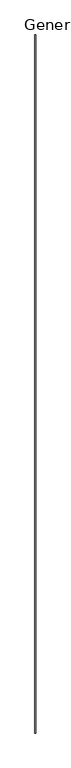
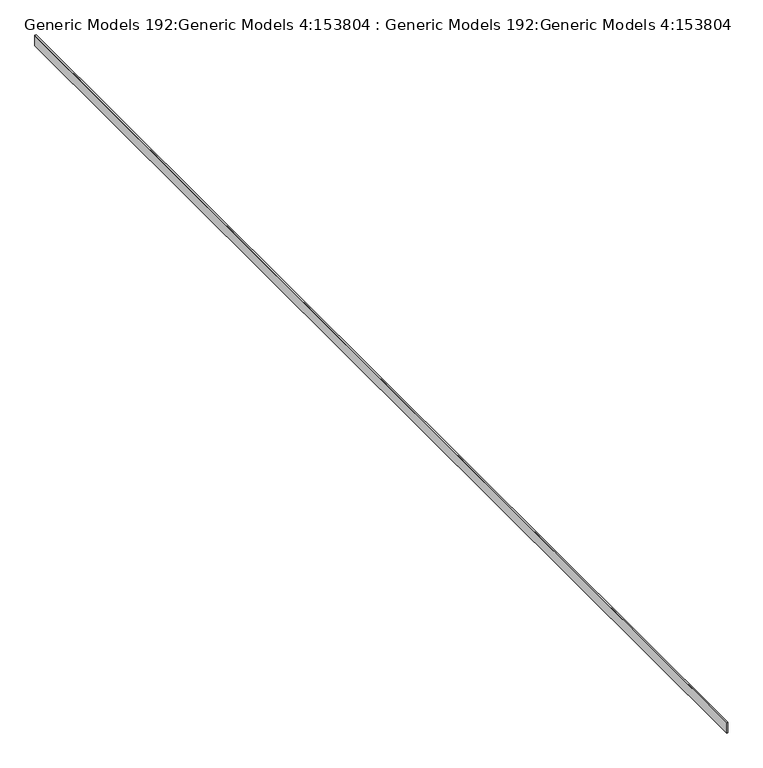
"""IFC4 building model written with IfcOpenShell, lengths in millimetres: proxy geometry, Generic Models 192:Generic Models 4:153804 : Generic Models 192:Generic Models 4:153804."""

import ifcopenshell
import ifcopenshell.guid

model = None  # the IFC model being written
_history = None  # IfcOwnerHistory: only IFC2X3 demands one
_inside = {}  # id of a spatial element -> (the spatial element, [elements in it])
_under = {}  # id of a project, library or spatial element -> (it, [spatial elements below it])
_declared = {}  # id of a project -> (the project, [libraries it declares])
_typed = {}  # id of a type object -> (the type object, [elements of that type])
_made_of = {}  # id of a material, layer set ... -> (it, [elements and type objects made of it])


def new_model(schema):
    """Start an empty IFC model of exactly this schema.

    Asked for "IFC4X3", IfcOpenShell would pick the latest addendum, in which some entities
    have other attributes; the version numbers below select the first issue.
    IFC2X3 requires an IfcOwnerHistory on every rooted entity: one is made here for all.
    """
    global model, _history
    if schema == "IFC4X3":
        model = ifcopenshell.file(schema_version=(4, 3, 0, 0))
    else:
        model = ifcopenshell.file(schema=schema)
    _inside.clear()
    _under.clear()
    _declared.clear()
    _typed.clear()
    _made_of.clear()
    _history = None
    if model.schema == "IFC2X3":
        org = make("IfcOrganization", Name="unknown")
        user = make(
            "IfcPersonAndOrganization",
            ThePerson=make("IfcPerson", FamilyName="unknown"),
            TheOrganization=org,
        )
        app = make(
            "IfcApplication",
            ApplicationDeveloper=org,
            Version="unknown",
            ApplicationFullName="unknown",
            ApplicationIdentifier="unknown",
        )
        _history = make(
            "IfcOwnerHistory",
            OwningUser=user,
            OwningApplication=app,
            ChangeAction="ADDED",
            CreationDate=0,
        )
    return model


def make(cls, **values):
    """One entity of the class cls with the attributes given. An attribute that is None is left unset."""
    return model.create_entity(
        cls, **{name: value for name, value in values.items() if value is not None}
    )


def rooted(cls, **values):
    """An entity with a GlobalId (a new one), such as an element, a storey or a relation."""
    return make(cls, GlobalId=ifcopenshell.guid.new(), OwnerHistory=_history, **values)


def si_unit(unit_type, name, prefix=None):
    """IfcSIUnit, for example si_unit("LENGTHUNIT", "METRE", prefix="MILLI")."""
    return make("IfcSIUnit", UnitType=unit_type, Prefix=prefix, Name=name)


def assignment(units):
    """IfcUnitAssignment: the units of a project."""
    return None if units is None else make("IfcUnitAssignment", Units=units)


def point(xyz):
    """IfcCartesianPoint."""
    return None if xyz is None else make("IfcCartesianPoint", Coordinates=xyz)


def direction(xyz):
    """IfcDirection."""
    return None if xyz is None else make("IfcDirection", DirectionRatios=xyz)


def frame(location, z_axis=None, x_axis=None):
    """IfcAxis2Placement3D, a coordinate frame: its origin and axes. An axis left out is left unset."""
    return make(
        "IfcAxis2Placement3D",
        Location=point(location),
        Axis=direction(z_axis),
        RefDirection=direction(x_axis),
    )


def origin():
    """The frame at (0, 0, 0) with its axes left unset."""
    return frame((0.0, 0.0, 0.0))


def place(relative_to, where):
    """IfcLocalPlacement: puts the frame where relative to a parent placement (None: the world)."""
    return make(
        "IfcLocalPlacement", PlacementRelTo=relative_to, RelativePlacement=where
    )


def context(
    kind, dimensions, precision=None, world=None, true_north=None, identifier=None
):
    """IfcGeometricRepresentationContext, for example the 3D "Model" context."""
    return make(
        "IfcGeometricRepresentationContext",
        ContextIdentifier=identifier,
        ContextType=kind,
        CoordinateSpaceDimension=dimensions,
        Precision=precision,
        WorldCoordinateSystem=world,
        TrueNorth=true_north,
    )


def project(units=None, contexts=None):
    """IfcProject with its units and contexts."""
    return rooted(
        "IfcProject",
        Name="project",
        RepresentationContexts=contexts,
        UnitsInContext=assignment(units),
    )


def spatial(cls, under=None, at=None, **own):
    """A site, building, storey or space (cls), placed at a placement, below another one or the project."""
    s = rooted(cls, ObjectPlacement=at, **own)
    if under is not None:
        _under.setdefault(under.id(), (under, []))[1].append(s)
    return s


def polyline(points):
    """IfcPolyline through the points."""
    return make("IfcPolyline", Points=[point(p) for p in points])


def outline(outer, holes=None, kind="AREA"):
    """IfcArbitraryClosedProfileDef: a profile drawn as a closed curve; with holes, ...WithVoids."""
    if holes is None:
        return make("IfcArbitraryClosedProfileDef", ProfileType=kind, OuterCurve=outer)
    return make(
        "IfcArbitraryProfileDefWithVoids",
        ProfileType=kind,
        OuterCurve=outer,
        InnerCurves=holes,
    )


def extrude(swept, where, along, depth):
    """IfcExtrudedAreaSolid: the profile swept, set in the frame where, extruded along a direction by depth."""
    return make(
        "IfcExtrudedAreaSolid",
        SweptArea=swept,
        Position=where,
        ExtrudedDirection=direction(along),
        Depth=depth,
    )


def shape(context_of_items, identifier, shape_type, items):
    """IfcShapeRepresentation: the items that make up one representation, for example the "Body"."""
    return make(
        "IfcShapeRepresentation",
        ContextOfItems=context_of_items,
        RepresentationIdentifier=identifier,
        RepresentationType=shape_type,
        Items=items,
    )


def source(mapping_origin, context_of_items, identifier, shape_type, items):
    """IfcRepresentationMap: a shape defined once, which mapped items show again and again."""
    return make(
        "IfcRepresentationMap",
        MappingOrigin=mapping_origin,
        MappedRepresentation=shape(context_of_items, identifier, shape_type, items),
    )


def transform(
    local_origin,
    x_axis=None,
    y_axis=None,
    z_axis=None,
    scale=None,
    scale2=None,
    scale3=None,
    uniform=True,
):
    """IfcCartesianTransformationOperator3D, or its non-uniform kind. x_axis, y_axis, z_axis: its Axis1, 2, 3."""
    if uniform:
        return make(
            "IfcCartesianTransformationOperator3D",
            Axis1=direction(x_axis),
            Axis2=direction(y_axis),
            LocalOrigin=point(local_origin),
            Scale=scale,
            Axis3=direction(z_axis),
        )
    return make(
        "IfcCartesianTransformationOperator3DnonUniform",
        Axis1=direction(x_axis),
        Axis2=direction(y_axis),
        LocalOrigin=point(local_origin),
        Scale=scale,
        Axis3=direction(z_axis),
        Scale2=scale2,
        Scale3=scale3,
    )


def mapped(mapping_source, mapping_target):
    """IfcMappedItem: shows the shape of a source again, moved by a transform."""
    return make(
        "IfcMappedItem", MappingSource=mapping_source, MappingTarget=mapping_target
    )


def made_of(thing, what):
    """Note that an element or type object is made of a material, layer set ...; save() writes the relation."""
    if what is not None:
        _made_of.setdefault(what.id(), (what, []))[1].append(thing)
    return thing


def element(
    cls,
    number,
    at=None,
    inside=None,
    cuts=None,
    type_object=None,
    material=None,
    context=None,
    identifier="Body",
    shape_type=None,
    held_by="IfcProductDefinitionShape",
    body=None,
    shapes=None,
    **own,
):
    """One element of the class cls, such as IfcWall. Its Tag is "e" and its number.

    at: its placement. inside: the storey or other place that contains it. cuts: it is an
    opening in that element (IfcRelVoidsElement). A single representation is given by context,
    identifier, shape_type and body (its items); several are given by shapes. held_by: the class
    of the entity that holds the representations. save() writes the other relations.
    """
    e = rooted(cls, Tag="e%d" % number, ObjectPlacement=at, **own)
    if body is not None:
        shapes = [shape(context, identifier, shape_type, body)]
    if shapes is not None:
        e.Representation = make(held_by, Representations=shapes)
    if inside is not None:
        _inside.setdefault(inside.id(), (inside, []))[1].append(e)
    if cuts is not None:
        rooted(
            "IfcRelVoidsElement", RelatingBuildingElement=cuts, RelatedOpeningElement=e
        )
    if type_object is not None:
        _typed.setdefault(type_object.id(), (type_object, []))[1].append(e)
    return made_of(e, material)


def aggregate(whole, parts):
    """IfcRelAggregates: a whole, such as a stair, and the parts it consists of."""
    return rooted("IfcRelAggregates", RelatingObject=whole, RelatedObjects=parts)


def save(model, path):
    """Write the relations noted so far, then the file.

    IfcRelAggregates (storeys below a building ...), IfcRelContainedInSpatialStructure (elements
    in a storey), IfcRelDefinesByType, IfcRelAssociatesMaterial and IfcRelDeclares: one each for
    every whole, place, type object, material and project.
    """
    for whole, parts in _under.values():
        aggregate(whole, parts)
    for where, things in _inside.values():
        rooted(
            "IfcRelContainedInSpatialStructure",
            RelatedElements=things,
            RelatingStructure=where,
        )
    for kind, things in _typed.values():
        rooted("IfcRelDefinesByType", RelatedObjects=things, RelatingType=kind)
    for what, things in _made_of.values():
        rooted("IfcRelAssociatesMaterial", RelatedObjects=things, RelatingMaterial=what)
    for by, libraries in _declared.values():
        rooted("IfcRelDeclares", RelatingContext=by, RelatedDefinitions=libraries)
    model.write(path)


def generic_models_192_generic_models_4_153804_generic_models_35be6b02(model_context):
    return source(origin(), model_context, "Body", "SweptSolid", [
        extrude(outline(polyline([(5887.8852308, -5397.0793913), (5887.8852308, -5378.7594166), (6059.882074, -5378.7594166), (6059.882074, -5395.8093913), (6056.402274, -5395.8093913), (6056.402274, -5397.0793913), (5887.8852308, -5397.0793913)])), frame((0.0, -6674.7974793, 0.0), z_axis=(0.0, 1.0, 0.0), x_axis=(0.0, 0.0, 1.0)), (0.0, 0.0, 1.0), 18643.6),
    ])


if __name__ == "__main__":
    model = new_model("IFC4")
    model_context = context("Model", 3, world=origin())
    ifc_project = project(units=[si_unit("LENGTHUNIT", "METRE", prefix="MILLI")], contexts=[model_context])
    site = spatial("IfcSite", under=ifc_project)
    building = spatial("IfcBuilding", under=site)
    placement = place(None, origin())
    generic_models_192_generic_models_4_153804_generic_models_shape = generic_models_192_generic_models_4_153804_generic_models_35be6b02(model_context)
    element("IfcBuildingElementProxy", 1, Name="Generic Models 192:Generic Models 4:153804 : Generic Models 192:Generic Models 4:153804", ObjectType="Generic Models 192:Generic Models 4:153804 : Generic Models 192:Generic Models 4:153804", at=placement, inside=building, context=model_context, shape_type="MappedRepresentation", body=[
        mapped(generic_models_192_generic_models_4_153804_generic_models_shape, transform((0.0, 0.0, 0.0), x_axis=(1.0, 0.0, 0.0), y_axis=(0.0, 1.0, 0.0), z_axis=(0.0, 0.0, 1.0))),
    ])
    save(model, "model.ifc")

# Revit data of these elements
# Type "Generic Models 192:Generic Models 4:153804 : Generic Models 192:Generic Models 4:153804"
#   NameOverride = "Generic Models 192:Generic Models 4:153804"
#   ObjectTypeOverride = "Generic Models 192:Generic Models 4"
#   Reference = "Generic Models 4"
#   Category = "Generic Models"
#   Tag = "153804"
# Element 1 (IfcBuildingElementProxy, "Generic Models 192:Generic Models 4:153804 : Generic Models 192:Generic Models 4:153804")
#   Materials on its faces: "_7/8\" SMOOTH TROWEL EXTERIOR STUCCO (COLOR PER OWNER) 770"
# Materials
#   "_7/8\" SMOOTH TROWEL EXTERIOR STUCCO (COLOR PER OWNER) 770": class "Unassigned", colour RGB 233 233 233, transparency 0
